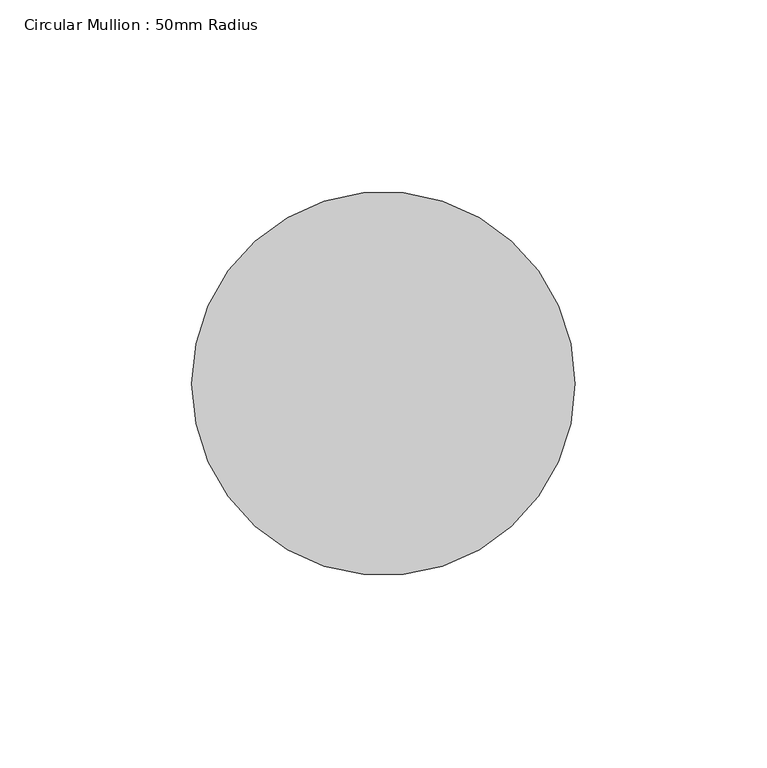
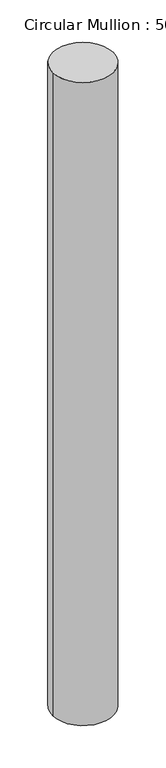
"""IFC4 building model written with IfcOpenShell, lengths in millimetres: member geometry, Circular Mullion : 50mm Radius."""

from ifc_helpers import new_model, si_unit, point, frame, origin, origin_2d, place, context, project, spatial, circle_curve, trimmed, segment, composite_curve, outline, extrude, source, transform, mapped, element, save


def circular_mullion_50mm_radius_c99b4bc9(model_context):
    return source(origin(), model_context, "Body", "SweptSolid", [
        extrude(outline(composite_curve([segment(trimmed(circle_curve(origin_2d(), 50.0), [point((50.0, 0.0))], [point((-50.0, 0.0))], False, "CARTESIAN"), True, "CONTINUOUS"), segment(trimmed(circle_curve(origin_2d(), 50.0), [point((-50.0, 0.0))], [point((50.0, 0.0))], False, "CARTESIAN"), True, "CONTINUOUS")], self_intersect=False)), frame((0.0, 0.0, -1120.6798937), z_axis=(0.0, 0.0, 1.0), x_axis=(1.0, 0.0, 0.0)), (0.0, 0.0, 1.0), 1120.6798937),
    ])


if __name__ == "__main__":
    model = new_model("IFC4")
    model_context = context("Model", 3, world=origin())
    ifc_project = project(units=[si_unit("LENGTHUNIT", "METRE", prefix="MILLI")], contexts=[model_context])
    site = spatial("IfcSite", under=ifc_project)
    building = spatial("IfcBuilding", under=site)
    placement = place(None, origin())
    circular_mullion_50mm_radius_shape = circular_mullion_50mm_radius_c99b4bc9(model_context)
    element("IfcMember", 1, ObjectType="Circular Mullion : 50mm Radius", at=placement, inside=building, context=model_context, shape_type="MappedRepresentation", body=[
        mapped(circular_mullion_50mm_radius_shape, transform((0.0, 0.0, 0.0), x_axis=(1.0, 0.0, 0.0), y_axis=(0.0, 1.0, 0.0), z_axis=(0.0, 0.0, 1.0))),
    ])
    save(model, "model.ifc")

# Revit data of these elements
# Type "Circular Mullion : 50mm Radius"
#   built-in parameter 1007350 = 0.164042 (stored number, unit not read)
# Element 1 (IfcMember, "Circular Mullion : 50mm Radius")
#   Materials on its faces: "Aluminium"
# Materials
#   "Aluminium": class "Metal", colour RGB 247 247 247, transparency 0, Description = "Aluminium 6061", Cost = 0
